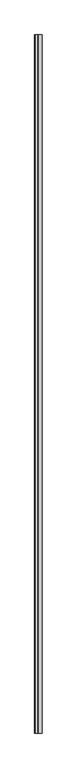
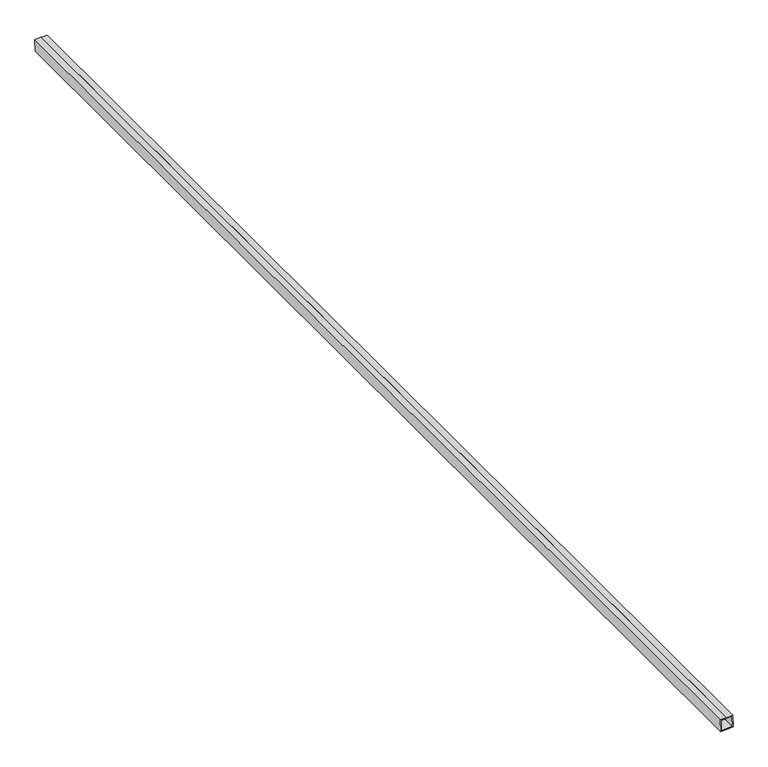
"""IFC4 building model written with IfcOpenShell, lengths in millimetres: proxy geometry, Inner panel:Inner panel:1:Inner panel:1 : Inner panel:Inner panel:300324:2:Inner panel:1:Inner panel:1 : Inner panel:Inner panel:300324:2 : Inner panel:Inner panel:1:Inner panel:1 : Inner panel:Inner panel:300324:300043:29 : Inner panel:Inner panel:1:Inner panel:1 : Inner panel:Inner panel:300324:2:Inner panel:1:Inner panel:1 : Inner panel:Inner panel:300324:2 : Inner panel:Inner panel:1:Inner panel:1 : Inner panel:Inner panel:300324:300043:308120."""

from ifc_helpers import new_model, si_unit, frame, origin, place, context, project, spatial, polyline, outline, extrude, source, transform, mapped, element, save


def generic_models_312fd8cf(model_context):
    return source(origin(), model_context, "Body", "SweptSolid", [
        extrude(outline(polyline([(3857.794365, 558155.1660493), (3855.4151794, 558155.265182), (3856.0760643, 558171.1264196), (3822.7674654, 558172.5142778), (3821.3796071, 558139.205679), (3854.688206, 558137.8178207), (3855.3490909, 558153.6790583), (3857.7282765, 558153.5799255), (3856.9682589, 558135.3395024), (3818.9012888, 558136.9256261), (3820.4874125, 558174.9925962), (3858.5543826, 558173.4064725), (3857.794365, 558155.1660493)])), frame((0.0, -579334.066384, 0.0), z_axis=(0.0, 1.0, 0.0), x_axis=(0.0, 0.0, 1.0)), (0.0, 0.0, 1.0), 3657.6),
    ])


if __name__ == "__main__":
    model = new_model("IFC4")
    model_context = context("Model", 3, world=origin())
    ifc_project = project(units=[si_unit("LENGTHUNIT", "METRE", prefix="MILLI")], contexts=[model_context])
    site = spatial("IfcSite", under=ifc_project)
    building = spatial("IfcBuilding", under=site)
    placement = place(None, origin())
    generic_models_shape = generic_models_312fd8cf(model_context)
    element("IfcBuildingElementProxy", 1, Name="Inner panel:Inner panel:1:Inner panel:1 : Inner panel:Inner panel:300324:2:Inner panel:1:Inner panel:1 : Inner panel:Inner panel:300324:2 : Inner panel:Inner panel:1:Inner panel:1 : Inner panel:Inner panel:300324:300043:29 : Inner panel:Inner panel:1:Inner panel:1 : Inner panel:Inner panel:300324:2:Inner panel:1:Inner panel:1 : Inner panel:Inner panel:300324:2 : Inner panel:Inner panel:1:Inner panel:1 : Inner panel:Inner panel:300324:300043:308120", ObjectType="Inner panel:Inner panel:1:Inner panel:1 : Inner panel:Inner panel:300324:2:Inner panel:1:Inner panel:1 : Inner panel:Inner panel:300324:2 : Inner panel:Inner panel:1:Inner panel:1 : Inner panel:Inner panel:300324:300043:29 : Inner panel:Inner panel:1:Inner panel:1 : Inner panel:Inner panel:300324:2:Inner panel:1:Inner panel:1 : Inner panel:Inner panel:300324:2 : Inner panel:Inner panel:1:Inner panel:1 : Inner panel:Inner panel:300324:300043:308120", at=placement, inside=building, context=model_context, shape_type="MappedRepresentation", body=[
        mapped(generic_models_shape, transform((0.0, 0.0, 0.0), x_axis=(1.0, 0.0, 0.0), y_axis=(0.0, 1.0, 0.0), z_axis=(0.0, 0.0, 1.0))),
    ])
    save(model, "model.ifc")

# Revit data of these elements
# Type "Inner panel:Inner panel:1:Inner panel:1 : Inner panel:Inner panel:300324:2:Inner panel:1:Inner panel:1 : Inner panel:Inner panel:300324:2 : Inner panel:Inner panel:1:Inner panel:1 : Inner panel:Inner panel:300324:300043:29 : Inner panel:Inner panel:1:Inner panel:1 : Inner panel:Inner panel:300324:2:Inner panel:1:Inner panel:1 : Inner panel:Inner panel:300324:2 : Inner panel:Inner panel:1:Inner panel:1 : Inner panel:Inner panel:300324:300043:308120"
#   NameOverride = "Inner panel:Inner panel:1:Inner panel:1 : Inner panel:Inner panel:300324:2:Inner panel:1:Inner panel:1 : Inner panel:Inner panel:300324:2 : Inner panel:Inner panel:1:Inner panel:1 : Inner panel:Inner panel:300324:300043:308120"
#   ObjectTypeOverride = "Inner panel:1:Inner panel:1 : Inner panel:Inner panel:300324:2 : Inner panel:Inner panel:1:Inner panel:1 : Inner panel:Inner panel:300324:300043"
#   Reference = "Inner panel"
#   Tag = "308120"
# Element 1 (IfcBuildingElementProxy, "Inner panel:Inner panel:1:Inner panel:1 : Inner panel:Inner panel:300324:2:Inner panel:1:Inner panel:1 : Inner panel:Inner panel:300324:2 : Inner panel:Inner panel:1:Inner panel:1 : Inner panel:Inner panel:300324:300043:29 : Inner panel:Inner panel:1:Inner panel:1 : Inner panel:Inner panel:300324:2:Inner panel:1:Inner panel:1 : Inner panel:Inner panel:300324:2 : Inner panel:Inner panel:1:Inner panel:1 : Inner panel:Inner panel:300324:300043:308120")
#   Materials on its faces: "1 1/2\" X 1 1/2\" SPLIT-SEAM SQUARE TUBING (~24\" CANTILEVER FROM C.L. OF GLULAM)"
# Materials
#   "1 1/2\" X 1 1/2\" SPLIT-SEAM SQUARE TUBING (~24\" CANTILEVER FROM C.L. OF GLULAM)": class "Unassigned", colour RGB 202 201 200, transparency 0, Cost = 0
